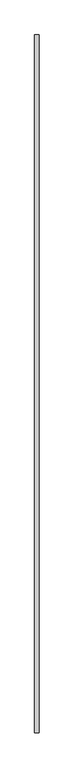
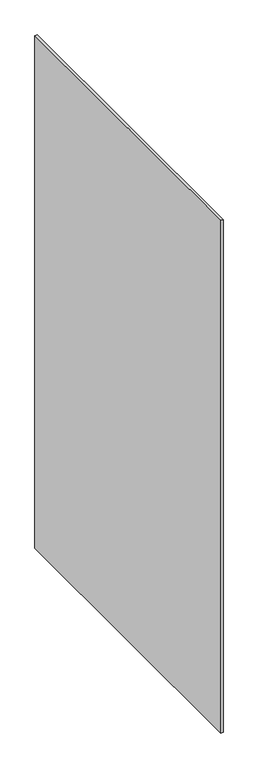
"""IFC4 building model written with IfcOpenShell, lengths in millimetres: proxy geometry, Panel:Panel:300402:Panel:300402 : Panel:Panel:300402:300124:Panel:300402:Panel:300402 : Panel:Panel:300402:300124 : Panel:Panel:300402:Panel:300402 : Panel:Panel:300402:300124:9 : Panel:Panel:300402:Panel:300402 : Panel:Panel:300402:300124:Panel:300402:Panel:300402 : Panel:Panel:300402:300124 : Panel:Panel:300402:Panel:300402 : Panel:Panel:300402:300124:300083."""

from ifc_helpers import new_model, si_unit, frame, origin, place, context, project, spatial, polyline, outline, extrude, source, transform, mapped, element, save


def generic_models_ebaa359b(model_context):
    return source(origin(), model_context, "Body", "SweptSolid", [
        extrude(outline(polyline([(579383.9117239, -577498.9163841), (579391.8492239, -577498.9163841), (579391.8492239, -578718.1163841), (579383.9117239, -578718.1163841), (579383.9117239, -577498.9163841)])), frame((0.0, 0.0, 4090.9180198), z_axis=(0.0, 0.0, 1.0), x_axis=(1.0, 0.0, 0.0)), (0.0, 0.0, 1.0), 2050.7302097),
    ])


if __name__ == "__main__":
    model = new_model("IFC4")
    model_context = context("Model", 3, world=origin())
    ifc_project = project(units=[si_unit("LENGTHUNIT", "METRE", prefix="MILLI")], contexts=[model_context])
    site = spatial("IfcSite", under=ifc_project)
    building = spatial("IfcBuilding", under=site)
    placement = place(None, origin())
    generic_models_shape = generic_models_ebaa359b(model_context)
    element("IfcBuildingElementProxy", 1, Name="Panel:Panel:300402:Panel:300402 : Panel:Panel:300402:300124:Panel:300402:Panel:300402 : Panel:Panel:300402:300124 : Panel:Panel:300402:Panel:300402 : Panel:Panel:300402:300124:9 : Panel:Panel:300402:Panel:300402 : Panel:Panel:300402:300124:Panel:300402:Panel:300402 : Panel:Panel:300402:300124 : Panel:Panel:300402:Panel:300402 : Panel:Panel:300402:300124:300083", ObjectType="Panel:Panel:300402:Panel:300402 : Panel:Panel:300402:300124:Panel:300402:Panel:300402 : Panel:Panel:300402:300124 : Panel:Panel:300402:Panel:300402 : Panel:Panel:300402:300124:9 : Panel:Panel:300402:Panel:300402 : Panel:Panel:300402:300124:Panel:300402:Panel:300402 : Panel:Panel:300402:300124 : Panel:Panel:300402:Panel:300402 : Panel:Panel:300402:300124:300083", at=placement, inside=building, context=model_context, shape_type="MappedRepresentation", body=[
        mapped(generic_models_shape, transform((0.0, 0.0, 0.0), x_axis=(1.0, 0.0, 0.0), y_axis=(0.0, 1.0, 0.0), z_axis=(0.0, 0.0, 1.0))),
    ])
    save(model, "model.ifc")

# Revit data of these elements
# Type "Panel:Panel:300402:Panel:300402 : Panel:Panel:300402:300124:Panel:300402:Panel:300402 : Panel:Panel:300402:300124 : Panel:Panel:300402:Panel:300402 : Panel:Panel:300402:300124:9 : Panel:Panel:300402:Panel:300402 : Panel:Panel:300402:300124:Panel:300402:Panel:300402 : Panel:Panel:300402:300124 : Panel:Panel:300402:Panel:300402 : Panel:Panel:300402:300124:300083"
#   NameOverride = "Panel:Panel:300402:Panel:300402 : Panel:Panel:300402:300124:Panel:300402:Panel:300402 : Panel:Panel:300402:300124 : Panel:Panel:300402:Panel:300402 : Panel:Panel:300402:300124:300083"
#   ObjectTypeOverride = "Panel:300402:Panel:300402 : Panel:Panel:300402:300124 : Panel:Panel:300402:Panel:300402 : Panel:Panel:300402:300124"
#   Reference = "Panel"
#   Tag = "300083"
# Element 1 (IfcBuildingElementProxy, "Panel:Panel:300402:Panel:300402 : Panel:Panel:300402:300124:Panel:300402:Panel:300402 : Panel:Panel:300402:300124 : Panel:Panel:300402:Panel:300402 : Panel:Panel:300402:300124:9 : Panel:Panel:300402:Panel:300402 : Panel:Panel:300402:300124:Panel:300402:Panel:300402 : Panel:Panel:300402:300124 : Panel:Panel:300402:Panel:300402 : Panel:Panel:300402:300124:300083")
#   Materials on its faces: "5/16\" PHENOLIC RESIN PANELS (CLASS A FLAME SPREAD) - EXPOSED FASTENERS"
# Materials
#   "5/16\" PHENOLIC RESIN PANELS (CLASS A FLAME SPREAD) - EXPOSED FASTENERS": class "Unassigned", colour RGB 64 64 64, transparency 0, Keynote = "M07420000.01", Cost = 0
